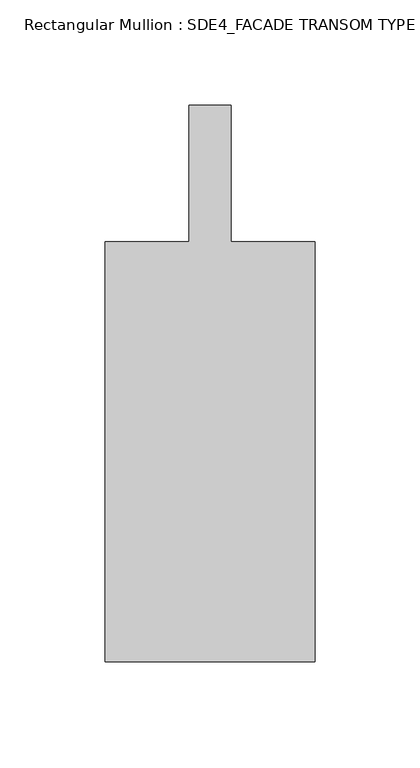
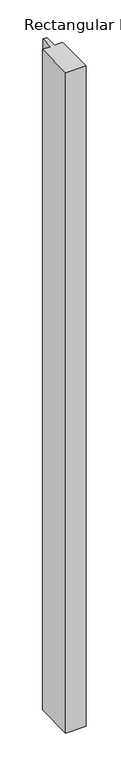
"""IFC4 building model written with IfcOpenShell, lengths in millimetres: member geometry, Rectangular Mullion : SDE4_FACADE TRANSOM TYPE 2."""

from ifc_helpers import new_model, si_unit, frame, origin, place, context, project, spatial, polyline, outline, extrude, source, transform, mapped, element, save


def rectangular_mullion_sde4_facade_transom_type_2_3499d9fb(model_context):
    return source(origin(), model_context, "Body", "SweptSolid", [
        extrude(outline(polyline([(50.0, -132.5), (-50.0, -132.5), (-50.0, 67.5), (-10.0, 67.5), (-10.0, 132.5), (10.0, 132.5), (10.0, 67.5), (50.0, 67.5), (50.0, -132.5)])), frame((0.0, 0.0, -3439.0), z_axis=(0.0, 0.0, 1.0), x_axis=(1.0, 0.0, 0.0)), (0.0, 0.0, 1.0), 3439.0),
    ])


if __name__ == "__main__":
    model = new_model("IFC4")
    model_context = context("Model", 3, world=origin())
    ifc_project = project(units=[si_unit("LENGTHUNIT", "METRE", prefix="MILLI")], contexts=[model_context])
    site = spatial("IfcSite", under=ifc_project)
    building = spatial("IfcBuilding", under=site)
    placement = place(None, origin())
    rectangular_mullion_sde4_facade_transom_type_2_shape = rectangular_mullion_sde4_facade_transom_type_2_3499d9fb(model_context)
    element("IfcMember", 1, ObjectType="Rectangular Mullion : SDE4_FACADE TRANSOM TYPE 2", at=placement, inside=building, context=model_context, shape_type="MappedRepresentation", body=[
        mapped(rectangular_mullion_sde4_facade_transom_type_2_shape, transform((0.0, 0.0, 0.0), x_axis=(1.0, 0.0, 0.0), y_axis=(0.0, 1.0, 0.0), z_axis=(0.0, 0.0, 1.0))),
    ])
    save(model, "model.ifc")

# Revit data of these elements
# Type "Rectangular Mullion : SDE4_FACADE TRANSOM TYPE 2"
#   built-in parameter 1007322 = 0.869423 (stored number, unit not read)
#   built-in parameter 1007321 = 0.164042 (stored number, unit not read)
#   built-in parameter 1007320 = 0.164042 (stored number, unit not read)
